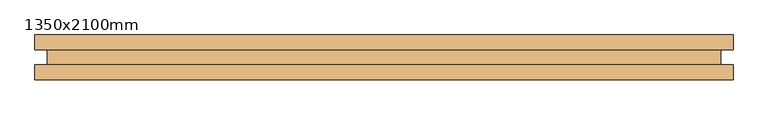
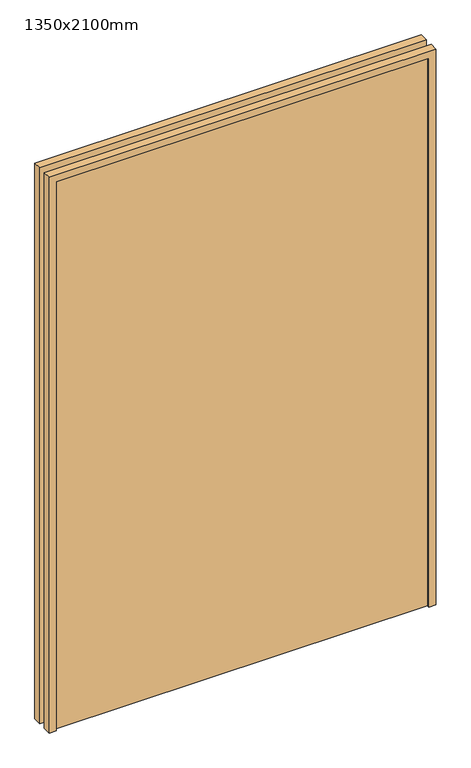
"""IFC4 building model written with IfcOpenShell, lengths in millimetres: door geometry, WWm-SingleSolid-Flush : 1350x2100mm."""

from ifc_helpers import new_model, si_unit, frame, origin, origin_with_axes, place, context, project, spatial, polyline, outline, extrude, source, transform, mapped, element, save


def door_1350x2100mm_132f6529(model_context):
    return source(origin(), model_context, "Body", "SweptSolid", [
        extrude(outline(polyline([(2125.0, -700.0), (0.0, -700.0), (0.0, -675.0), (2100.0, -675.0), (2100.0, 675.0), (0.0, 675.0), (0.0, 700.0), (2125.0, 700.0), (2125.0, -700.0)])), frame((0.0, 15.0, 0.0), z_axis=(0.0, 1.0, 0.0), x_axis=(0.0, 0.0, 1.0)), (0.0, 0.0, 1.0), 30.0),
        extrude(outline(polyline([(2125.0, 700.0), (2125.0, -700.0), (0.0, -700.0), (0.0, -675.0), (2100.0, -675.0), (2100.0, 675.0), (0.0, 675.0), (0.0, 700.0), (2125.0, 700.0)])), frame((0.0, -45.0, 0.0), z_axis=(0.0, 1.0, 0.0), x_axis=(0.0, 0.0, 1.0)), (0.0, 0.0, 1.0), 30.0),
        extrude(outline(polyline([(675.0, -35.0), (-675.0, -35.0), (-675.0, 15.0), (675.0, 15.0), (675.0, -35.0)])), origin_with_axes(), (0.0, 0.0, 1.0), 2100.0),
    ])


if __name__ == "__main__":
    model = new_model("IFC4")
    model_context = context("Model", 3, world=origin())
    ifc_project = project(units=[si_unit("LENGTHUNIT", "METRE", prefix="MILLI")], contexts=[model_context])
    site = spatial("IfcSite", under=ifc_project)
    building = spatial("IfcBuilding", under=site)
    placement = place(None, origin())
    door_1350x2100mm_shape = door_1350x2100mm_132f6529(model_context)
    element("IfcDoor", 1, ObjectType="WWm-SingleSolid-Flush : 1350x2100mm", at=placement, inside=building, context=model_context, shape_type="MappedRepresentation", body=[
        mapped(door_1350x2100mm_shape, transform((0.0, 0.0, 0.0), x_axis=(1.0, 0.0, 0.0), y_axis=(0.0, 1.0, 0.0), z_axis=(0.0, 0.0, 1.0))),
    ])
    save(model, "model.ifc")

# Revit data of these elements
# Type "WWm-SingleSolid-Flush : 1350x2100mm"
#   Type Mark = "EX1-57"
#   Construction Type Id = "MDOOR"
#   Assembly Code = "C1020"
#   Analytic Construction = "Metal"
#   Thickness = 50 mm
#   Thermal Resistance (R) = 0.270117 (m²·K)/W
#   Heat Transfer Coefficient (U) = 3.7021 W/(m²·K)
#   Height = 2100 mm
#   Trim Projection Ext = 30 mm
#   Trim Projection Int = 30 mm
#   Trim Width = 25 mm
#   Width = 1350 mm
#   Not 90 Degree [instance default] = no
#   90 Degree [instance default] = yes
#   Door Material = WW-EC-RGB-White
#   Frame Material = WW-EC-RGB-White
#   Visual Light Transmittance = 0
#   Solar Heat Gain Coefficient = 0
#   Function = (empty or 0)
#   Wall Closure = (empty or 0)
# Element 1 (IfcDoor, "WWm-SingleSolid-Flush : 1350x2100mm")
#   Materials on its faces: "WW-EC-RGB-White"
# Materials
#   "WW-EC-RGB-White": class "Generic", colour RGB 255 255 255, transparency 0, Comments = "If region requests off-white, swith asset color to RGB 231-228-220", Description = "Generic Color", Cost = 0
